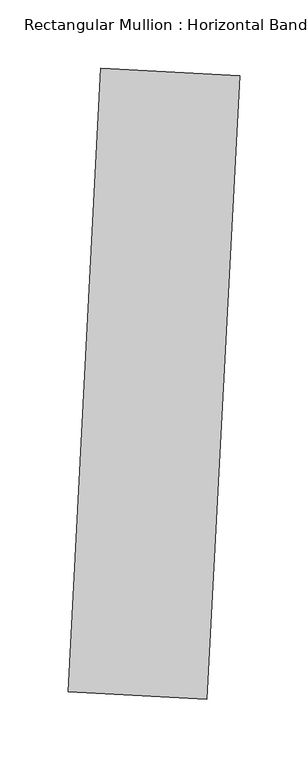
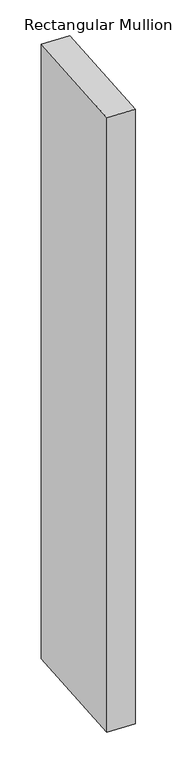
"""IFC4 building model written with IfcOpenShell, lengths in millimetres: member geometry, Rectangular Mullion : Horizontal Band."""

from ifc_helpers import new_model, si_unit, frame, origin, place, context, project, spatial, polyline, outline, extrude, source, transform, mapped, element, save


def rectangular_mullion_horizontal_band_f074a7b8(model_context):
    return source(origin(), model_context, "Body", "SweptSolid", [
        extrude(outline(polyline([(62.69438, 301.8280451), (38.7663808, -154.7453782), (-62.69438, -149.4280451), (-38.7663808, 307.1453782), (62.69438, 301.8280451)])), frame((0.0, 0.0, -2382.029342), z_axis=(0.0, 0.0, 1.0), x_axis=(1.0, 0.0, 0.0)), (0.0, 0.0, 1.0), 2382.029342),
    ])


if __name__ == "__main__":
    model = new_model("IFC4")
    model_context = context("Model", 3, world=origin())
    ifc_project = project(units=[si_unit("LENGTHUNIT", "METRE", prefix="MILLI")], contexts=[model_context])
    site = spatial("IfcSite", under=ifc_project)
    building = spatial("IfcBuilding", under=site)
    placement = place(None, origin())
    rectangular_mullion_horizontal_band_shape = rectangular_mullion_horizontal_band_f074a7b8(model_context)
    element("IfcMember", 1, ObjectType="Rectangular Mullion : Horizontal Band", at=placement, inside=building, context=model_context, shape_type="MappedRepresentation", body=[
        mapped(rectangular_mullion_horizontal_band_shape, transform((0.0, 0.0, 0.0), x_axis=(1.0, 0.0, 0.0), y_axis=(0.0, 1.0, 0.0), z_axis=(0.0, 0.0, 1.0))),
    ])
    save(model, "model.ifc")

# Revit data of these elements
# Type "Rectangular Mullion : Horizontal Band"
#   built-in parameter 1007351 = 0.25 (stored number, unit not read)
#   built-in parameter 1007304 = 1.5 (stored number, unit not read)
#   built-in parameter 1007301 = 0.166667 (stored number, unit not read)
#   built-in parameter 1007300 = 0.166667 (stored number, unit not read)
# Element 1 (IfcMember, "Rectangular Mullion : Horizontal Band")
#   Materials on its faces: "Aluminum"
# Materials
#   "Aluminum": class "Metal", colour RGB 247 247 247, transparency 0, Description = "Aluminum 6061", Cost = 0
